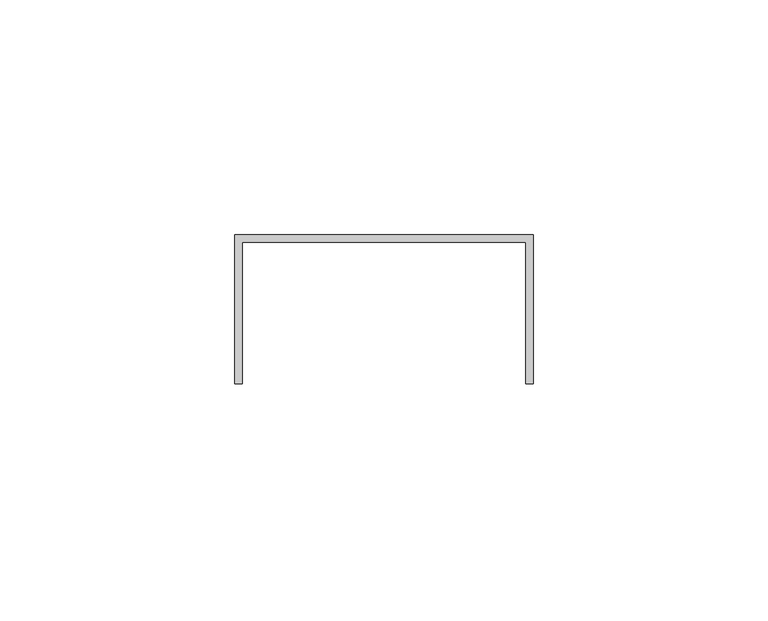
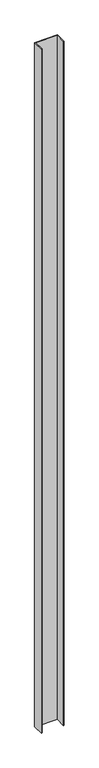
"""IFC4 building model written with IfcOpenShell, lengths in millimetres: proxy geometry, Generic Models 7:Generic Models 1:3:Generic Models 1:3 : Generic Models 7:Generic Models 1:305549:3:Generic Models 1:3:Generic Models 1:3 : Generic Models 7:Generic Models 1:305549:3 : Generic Models 7:Generic Models 1:3:Generic Models 1:3 : Generic Models 7:Generic Models 1:305549:301244:18 : Generic Models 7:Generic Models 1:3:Generic Models 1:3 : Generic Models 7:Generic Models 1:305549:3:Generic Models 1:3:Generic Models 1:3 : Generic Models 7:Generic Models 1:305549:3 : Generic Models 7:Generic Models 1:3:Generic Models 1:3 : Generic Models 7:Generic Models 1:305549:301244:308848."""

from ifc_helpers import new_model, si_unit, frame, origin, place, context, project, spatial, polyline, outline, extrude, source, transform, mapped, element, save


def generic_models_f29a7b32(model_context):
    return source(origin(), model_context, "Body", "SweptSolid", [
        extrude(outline(polyline([(560352.9617239, -578651.5664975), (560352.9617239, -578683.3164975), (560351.3742239, -578683.3164975), (560351.3742239, -578653.1539975), (560291.0492239, -578653.1539975), (560291.0492239, -578683.3164975), (560289.4617239, -578683.3164975), (560289.4617239, -578651.5664975), (560352.9617239, -578651.5664975)])), frame((0.0, 0.0, 4133.81326), z_axis=(0.0, 0.0, 1.0), x_axis=(1.0, 0.0, 0.0)), (0.0, 0.0, 1.0), 2000.28674),
    ])


if __name__ == "__main__":
    model = new_model("IFC4")
    model_context = context("Model", 3, world=origin())
    ifc_project = project(units=[si_unit("LENGTHUNIT", "METRE", prefix="MILLI")], contexts=[model_context])
    site = spatial("IfcSite", under=ifc_project)
    building = spatial("IfcBuilding", under=site)
    placement = place(None, origin())
    generic_models_shape = generic_models_f29a7b32(model_context)
    element("IfcBuildingElementProxy", 1, Name="Generic Models 7:Generic Models 1:3:Generic Models 1:3 : Generic Models 7:Generic Models 1:305549:3:Generic Models 1:3:Generic Models 1:3 : Generic Models 7:Generic Models 1:305549:3 : Generic Models 7:Generic Models 1:3:Generic Models 1:3 : Generic Models 7:Generic Models 1:305549:301244:18 : Generic Models 7:Generic Models 1:3:Generic Models 1:3 : Generic Models 7:Generic Models 1:305549:3:Generic Models 1:3:Generic Models 1:3 : Generic Models 7:Generic Models 1:305549:3 : Generic Models 7:Generic Models 1:3:Generic Models 1:3 : Generic Models 7:Generic Models 1:305549:301244:308848", ObjectType="Generic Models 7:Generic Models 1:3:Generic Models 1:3 : Generic Models 7:Generic Models 1:305549:3:Generic Models 1:3:Generic Models 1:3 : Generic Models 7:Generic Models 1:305549:3 : Generic Models 7:Generic Models 1:3:Generic Models 1:3 : Generic Models 7:Generic Models 1:305549:301244:18 : Generic Models 7:Generic Models 1:3:Generic Models 1:3 : Generic Models 7:Generic Models 1:305549:3:Generic Models 1:3:Generic Models 1:3 : Generic Models 7:Generic Models 1:305549:3 : Generic Models 7:Generic Models 1:3:Generic Models 1:3 : Generic Models 7:Generic Models 1:305549:301244:308848", at=placement, inside=building, context=model_context, shape_type="MappedRepresentation", body=[
        mapped(generic_models_shape, transform((0.0, 0.0, 0.0), x_axis=(1.0, 0.0, 0.0), y_axis=(0.0, 1.0, 0.0), z_axis=(0.0, 0.0, 1.0))),
    ])
    save(model, "model.ifc")

# Revit data of these elements
# Type "Generic Models 7:Generic Models 1:3:Generic Models 1:3 : Generic Models 7:Generic Models 1:305549:3:Generic Models 1:3:Generic Models 1:3 : Generic Models 7:Generic Models 1:305549:3 : Generic Models 7:Generic Models 1:3:Generic Models 1:3 : Generic Models 7:Generic Models 1:305549:301244:18 : Generic Models 7:Generic Models 1:3:Generic Models 1:3 : Generic Models 7:Generic Models 1:305549:3:Generic Models 1:3:Generic Models 1:3 : Generic Models 7:Generic Models 1:305549:3 : Generic Models 7:Generic Models 1:3:Generic Models 1:3 : Generic Models 7:Generic Models 1:305549:301244:308848"
#   NameOverride = "Generic Models 7:Generic Models 1:3:Generic Models 1:3 : Generic Models 7:Generic Models 1:305549:3:Generic Models 1:3:Generic Models 1:3 : Generic Models 7:Generic Models 1:305549:3 : Generic Models 7:Generic Models 1:3:Generic Models 1:3 : Generic Models 7:Generic Models 1:305549:301244:308848"
#   ObjectTypeOverride = "Generic Models 1:3:Generic Models 1:3 : Generic Models 7:Generic Models 1:305549:3 : Generic Models 7:Generic Models 1:3:Generic Models 1:3 : Generic Models 7:Generic Models 1:305549:301244"
#   Reference = "Generic Models 1"
#   Tag = "308848"
# Element 1 (IfcBuildingElementProxy, "Generic Models 7:Generic Models 1:3:Generic Models 1:3 : Generic Models 7:Generic Models 1:305549:3:Generic Models 1:3:Generic Models 1:3 : Generic Models 7:Generic Models 1:305549:3 : Generic Models 7:Generic Models 1:3:Generic Models 1:3 : Generic Models 7:Generic Models 1:305549:301244:18 : Generic Models 7:Generic Models 1:3:Generic Models 1:3 : Generic Models 7:Generic Models 1:305549:3:Generic Models 1:3:Generic Models 1:3 : Generic Models 7:Generic Models 1:305549:3 : Generic Models 7:Generic Models 1:3:Generic Models 1:3 : Generic Models 7:Generic Models 1:305549:301244:308848")
#   Materials on its faces: "GALVANIZED U-CHANNEL (250T125-33)"
# Materials
#   "GALVANIZED U-CHANNEL (250T125-33)": class "Unassigned", colour RGB 202 201 200, transparency 0, Keynote = "M05451300.02", Cost = 0
